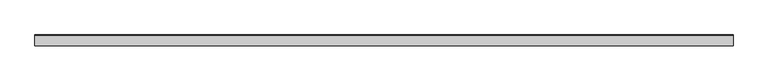
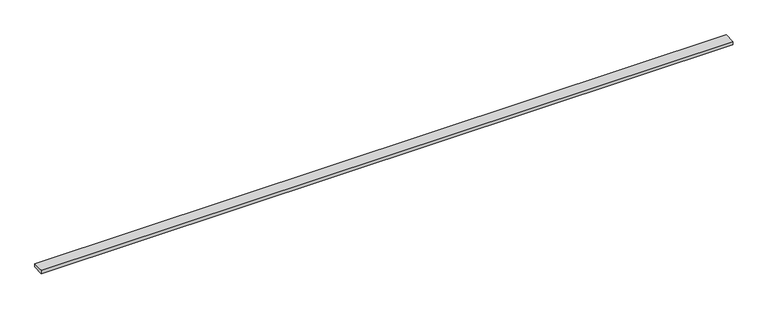
"""IFC4 building model written with IfcOpenShell, lengths in millimetres: proxy geometry, Inner panel:Inner panel:1:Inner panel:1 : Inner panel:Inner panel:300324:2:Inner panel:1:Inner panel:1 : Inner panel:Inner panel:300324:2 : Inner panel:Inner panel:1:Inner panel:1 : Inner panel:Inner panel:300324:300043:7 : Inner panel:Inner panel:1:Inner panel:1 : Inner panel:Inner panel:300324:2:Inner panel:1:Inner panel:1 : Inner panel:Inner panel:300324:2 : Inner panel:Inner panel:1:Inner panel:1 : Inner panel:Inner panel:300324:300043:308120."""

import ifcopenshell
import ifcopenshell.guid

model = None  # the IFC model being written
_history = None  # IfcOwnerHistory: only IFC2X3 demands one
_inside = {}  # id of a spatial element -> (the spatial element, [elements in it])
_under = {}  # id of a project, library or spatial element -> (it, [spatial elements below it])
_declared = {}  # id of a project -> (the project, [libraries it declares])
_typed = {}  # id of a type object -> (the type object, [elements of that type])
_made_of = {}  # id of a material, layer set ... -> (it, [elements and type objects made of it])


def new_model(schema):
    """Start an empty IFC model of exactly this schema.

    Asked for "IFC4X3", IfcOpenShell would pick the latest addendum, in which some entities
    have other attributes; the version numbers below select the first issue.
    IFC2X3 requires an IfcOwnerHistory on every rooted entity: one is made here for all.
    """
    global model, _history
    if schema == "IFC4X3":
        model = ifcopenshell.file(schema_version=(4, 3, 0, 0))
    else:
        model = ifcopenshell.file(schema=schema)
    _inside.clear()
    _under.clear()
    _declared.clear()
    _typed.clear()
    _made_of.clear()
    _history = None
    if model.schema == "IFC2X3":
        org = make("IfcOrganization", Name="unknown")
        user = make(
            "IfcPersonAndOrganization",
            ThePerson=make("IfcPerson", FamilyName="unknown"),
            TheOrganization=org,
        )
        app = make(
            "IfcApplication",
            ApplicationDeveloper=org,
            Version="unknown",
            ApplicationFullName="unknown",
            ApplicationIdentifier="unknown",
        )
        _history = make(
            "IfcOwnerHistory",
            OwningUser=user,
            OwningApplication=app,
            ChangeAction="ADDED",
            CreationDate=0,
        )
    return model


def make(cls, **values):
    """One entity of the class cls with the attributes given. An attribute that is None is left unset."""
    return model.create_entity(
        cls, **{name: value for name, value in values.items() if value is not None}
    )


def rooted(cls, **values):
    """An entity with a GlobalId (a new one), such as an element, a storey or a relation."""
    return make(cls, GlobalId=ifcopenshell.guid.new(), OwnerHistory=_history, **values)


def si_unit(unit_type, name, prefix=None):
    """IfcSIUnit, for example si_unit("LENGTHUNIT", "METRE", prefix="MILLI")."""
    return make("IfcSIUnit", UnitType=unit_type, Prefix=prefix, Name=name)


def assignment(units):
    """IfcUnitAssignment: the units of a project."""
    return None if units is None else make("IfcUnitAssignment", Units=units)


def point(xyz):
    """IfcCartesianPoint."""
    return None if xyz is None else make("IfcCartesianPoint", Coordinates=xyz)


def direction(xyz):
    """IfcDirection."""
    return None if xyz is None else make("IfcDirection", DirectionRatios=xyz)


def frame(location, z_axis=None, x_axis=None):
    """IfcAxis2Placement3D, a coordinate frame: its origin and axes. An axis left out is left unset."""
    return make(
        "IfcAxis2Placement3D",
        Location=point(location),
        Axis=direction(z_axis),
        RefDirection=direction(x_axis),
    )


def origin():
    """The frame at (0, 0, 0) with its axes left unset."""
    return frame((0.0, 0.0, 0.0))


def place(relative_to, where):
    """IfcLocalPlacement: puts the frame where relative to a parent placement (None: the world)."""
    return make(
        "IfcLocalPlacement", PlacementRelTo=relative_to, RelativePlacement=where
    )


def context(
    kind, dimensions, precision=None, world=None, true_north=None, identifier=None
):
    """IfcGeometricRepresentationContext, for example the 3D "Model" context."""
    return make(
        "IfcGeometricRepresentationContext",
        ContextIdentifier=identifier,
        ContextType=kind,
        CoordinateSpaceDimension=dimensions,
        Precision=precision,
        WorldCoordinateSystem=world,
        TrueNorth=true_north,
    )


def project(units=None, contexts=None):
    """IfcProject with its units and contexts."""
    return rooted(
        "IfcProject",
        Name="project",
        RepresentationContexts=contexts,
        UnitsInContext=assignment(units),
    )


def spatial(cls, under=None, at=None, **own):
    """A site, building, storey or space (cls), placed at a placement, below another one or the project."""
    s = rooted(cls, ObjectPlacement=at, **own)
    if under is not None:
        _under.setdefault(under.id(), (under, []))[1].append(s)
    return s


def polyline(points):
    """IfcPolyline through the points."""
    return make("IfcPolyline", Points=[point(p) for p in points])


def outline(outer, holes=None, kind="AREA"):
    """IfcArbitraryClosedProfileDef: a profile drawn as a closed curve; with holes, ...WithVoids."""
    if holes is None:
        return make("IfcArbitraryClosedProfileDef", ProfileType=kind, OuterCurve=outer)
    return make(
        "IfcArbitraryProfileDefWithVoids",
        ProfileType=kind,
        OuterCurve=outer,
        InnerCurves=holes,
    )


def extrude(swept, where, along, depth):
    """IfcExtrudedAreaSolid: the profile swept, set in the frame where, extruded along a direction by depth."""
    return make(
        "IfcExtrudedAreaSolid",
        SweptArea=swept,
        Position=where,
        ExtrudedDirection=direction(along),
        Depth=depth,
    )


def shape(context_of_items, identifier, shape_type, items):
    """IfcShapeRepresentation: the items that make up one representation, for example the "Body"."""
    return make(
        "IfcShapeRepresentation",
        ContextOfItems=context_of_items,
        RepresentationIdentifier=identifier,
        RepresentationType=shape_type,
        Items=items,
    )


def source(mapping_origin, context_of_items, identifier, shape_type, items):
    """IfcRepresentationMap: a shape defined once, which mapped items show again and again."""
    return make(
        "IfcRepresentationMap",
        MappingOrigin=mapping_origin,
        MappedRepresentation=shape(context_of_items, identifier, shape_type, items),
    )


def transform(
    local_origin,
    x_axis=None,
    y_axis=None,
    z_axis=None,
    scale=None,
    scale2=None,
    scale3=None,
    uniform=True,
):
    """IfcCartesianTransformationOperator3D, or its non-uniform kind. x_axis, y_axis, z_axis: its Axis1, 2, 3."""
    if uniform:
        return make(
            "IfcCartesianTransformationOperator3D",
            Axis1=direction(x_axis),
            Axis2=direction(y_axis),
            LocalOrigin=point(local_origin),
            Scale=scale,
            Axis3=direction(z_axis),
        )
    return make(
        "IfcCartesianTransformationOperator3DnonUniform",
        Axis1=direction(x_axis),
        Axis2=direction(y_axis),
        LocalOrigin=point(local_origin),
        Scale=scale,
        Axis3=direction(z_axis),
        Scale2=scale2,
        Scale3=scale3,
    )


def mapped(mapping_source, mapping_target):
    """IfcMappedItem: shows the shape of a source again, moved by a transform."""
    return make(
        "IfcMappedItem", MappingSource=mapping_source, MappingTarget=mapping_target
    )


def made_of(thing, what):
    """Note that an element or type object is made of a material, layer set ...; save() writes the relation."""
    if what is not None:
        _made_of.setdefault(what.id(), (what, []))[1].append(thing)
    return thing


def element(
    cls,
    number,
    at=None,
    inside=None,
    cuts=None,
    type_object=None,
    material=None,
    context=None,
    identifier="Body",
    shape_type=None,
    held_by="IfcProductDefinitionShape",
    body=None,
    shapes=None,
    **own,
):
    """One element of the class cls, such as IfcWall. Its Tag is "e" and its number.

    at: its placement. inside: the storey or other place that contains it. cuts: it is an
    opening in that element (IfcRelVoidsElement). A single representation is given by context,
    identifier, shape_type and body (its items); several are given by shapes. held_by: the class
    of the entity that holds the representations. save() writes the other relations.
    """
    e = rooted(cls, Tag="e%d" % number, ObjectPlacement=at, **own)
    if body is not None:
        shapes = [shape(context, identifier, shape_type, body)]
    if shapes is not None:
        e.Representation = make(held_by, Representations=shapes)
    if inside is not None:
        _inside.setdefault(inside.id(), (inside, []))[1].append(e)
    if cuts is not None:
        rooted(
            "IfcRelVoidsElement", RelatingBuildingElement=cuts, RelatedOpeningElement=e
        )
    if type_object is not None:
        _typed.setdefault(type_object.id(), (type_object, []))[1].append(e)
    return made_of(e, material)


def aggregate(whole, parts):
    """IfcRelAggregates: a whole, such as a stair, and the parts it consists of."""
    return rooted("IfcRelAggregates", RelatingObject=whole, RelatedObjects=parts)


def save(model, path):
    """Write the relations noted so far, then the file.

    IfcRelAggregates (storeys below a building ...), IfcRelContainedInSpatialStructure (elements
    in a storey), IfcRelDefinesByType, IfcRelAssociatesMaterial and IfcRelDeclares: one each for
    every whole, place, type object, material and project.
    """
    for whole, parts in _under.values():
        aggregate(whole, parts)
    for where, things in _inside.values():
        rooted(
            "IfcRelContainedInSpatialStructure",
            RelatedElements=things,
            RelatingStructure=where,
        )
    for kind, things in _typed.values():
        rooted("IfcRelDefinesByType", RelatedObjects=things, RelatingType=kind)
    for what, things in _made_of.values():
        rooted("IfcRelAssociatesMaterial", RelatedObjects=things, RelatingMaterial=what)
    for by, libraries in _declared.values():
        rooted("IfcRelDeclares", RelatingContext=by, RelatedDefinitions=libraries)
    model.write(path)


def generic_models_607a3d46(model_context):
    return source(origin(), model_context, "Body", "SweptSolid", [
        extrude(outline(polyline([(0.0, -75.8934963), (0.0, 0.0), (4876.8, 0.0), (4876.8, -75.8934963), (0.0, -75.8934963)])), frame((596182.8367239, -574602.2565563, 4107.7444302), z_axis=(0.0, -0.04163054471215047, 0.9991330730923532), x_axis=(-1.0, 0.0, 0.0)), (0.0, 0.0, 1.0), 25.4),
    ])


if __name__ == "__main__":
    model = new_model("IFC4")
    model_context = context("Model", 3, world=origin())
    ifc_project = project(units=[si_unit("LENGTHUNIT", "METRE", prefix="MILLI")], contexts=[model_context])
    site = spatial("IfcSite", under=ifc_project)
    building = spatial("IfcBuilding", under=site)
    placement = place(None, origin())
    generic_models_shape = generic_models_607a3d46(model_context)
    element("IfcBuildingElementProxy", 1, Name="Inner panel:Inner panel:1:Inner panel:1 : Inner panel:Inner panel:300324:2:Inner panel:1:Inner panel:1 : Inner panel:Inner panel:300324:2 : Inner panel:Inner panel:1:Inner panel:1 : Inner panel:Inner panel:300324:300043:7 : Inner panel:Inner panel:1:Inner panel:1 : Inner panel:Inner panel:300324:2:Inner panel:1:Inner panel:1 : Inner panel:Inner panel:300324:2 : Inner panel:Inner panel:1:Inner panel:1 : Inner panel:Inner panel:300324:300043:308120", ObjectType="Inner panel:Inner panel:1:Inner panel:1 : Inner panel:Inner panel:300324:2:Inner panel:1:Inner panel:1 : Inner panel:Inner panel:300324:2 : Inner panel:Inner panel:1:Inner panel:1 : Inner panel:Inner panel:300324:300043:7 : Inner panel:Inner panel:1:Inner panel:1 : Inner panel:Inner panel:300324:2:Inner panel:1:Inner panel:1 : Inner panel:Inner panel:300324:2 : Inner panel:Inner panel:1:Inner panel:1 : Inner panel:Inner panel:300324:300043:308120", at=placement, inside=building, context=model_context, shape_type="MappedRepresentation", body=[
        mapped(generic_models_shape, transform((0.0, 0.0, 0.0), x_axis=(1.0, 0.0, 0.0), y_axis=(0.0, 1.0, 0.0), z_axis=(0.0, 0.0, 1.0))),
    ])
    save(model, "model.ifc")

# Revit data of these elements
# Type "Inner panel:Inner panel:1:Inner panel:1 : Inner panel:Inner panel:300324:2:Inner panel:1:Inner panel:1 : Inner panel:Inner panel:300324:2 : Inner panel:Inner panel:1:Inner panel:1 : Inner panel:Inner panel:300324:300043:7 : Inner panel:Inner panel:1:Inner panel:1 : Inner panel:Inner panel:300324:2:Inner panel:1:Inner panel:1 : Inner panel:Inner panel:300324:2 : Inner panel:Inner panel:1:Inner panel:1 : Inner panel:Inner panel:300324:300043:308120"
#   NameOverride = "Inner panel:Inner panel:1:Inner panel:1 : Inner panel:Inner panel:300324:2:Inner panel:1:Inner panel:1 : Inner panel:Inner panel:300324:2 : Inner panel:Inner panel:1:Inner panel:1 : Inner panel:Inner panel:300324:300043:308120"
#   ObjectTypeOverride = "Inner panel:1:Inner panel:1 : Inner panel:Inner panel:300324:2 : Inner panel:Inner panel:1:Inner panel:1 : Inner panel:Inner panel:300324:300043"
#   Reference = "Inner panel"
#   Tag = "308120"
# Element 1 (IfcBuildingElementProxy, "Inner panel:Inner panel:1:Inner panel:1 : Inner panel:Inner panel:300324:2:Inner panel:1:Inner panel:1 : Inner panel:Inner panel:300324:2 : Inner panel:Inner panel:1:Inner panel:1 : Inner panel:Inner panel:300324:300043:7 : Inner panel:Inner panel:1:Inner panel:1 : Inner panel:Inner panel:300324:2:Inner panel:1:Inner panel:1 : Inner panel:Inner panel:300324:2 : Inner panel:Inner panel:1:Inner panel:1 : Inner panel:Inner panel:300324:300043:308120")
#   Materials on its faces: "1\" THERMAL SPACER @ PURLIN"
# Materials
#   "1\" THERMAL SPACER @ PURLIN": class "Unassigned", colour RGB 205 188 106, transparency 0, Cost = 0
